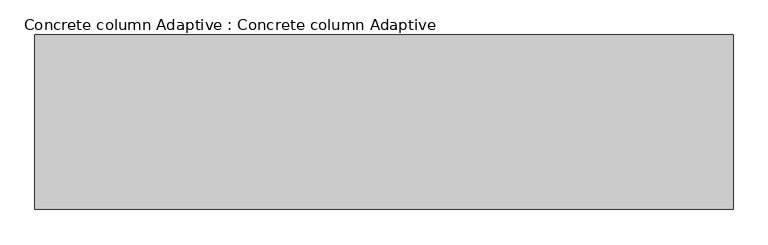
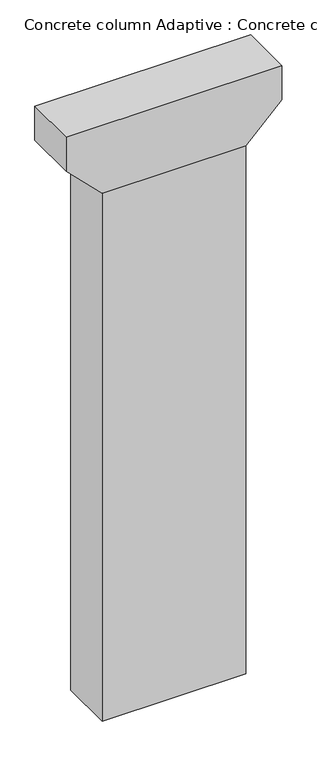
"""IFC4 building model written with IfcOpenShell, lengths in millimetres: proxy geometry, Concrete column Adaptive : Concrete column Adaptive."""

from ifc_helpers import new_model, si_unit, frame, origin, origin_with_axes, place, context, project, spatial, polyline, outline, extrude, source, transform, mapped, element, save


def concrete_column_adaptive_concrete_column_adaptive_b0f9f52a(model_context):
    return source(origin(), model_context, "Body", "SweptSolid", [
        extrude(outline(polyline([(35017.0, 6000.0), (35017.0, -6000.0), (33017.0, -6000.0), (31017.0, -4000.0), (31017.0, 4000.0), (33017.0, 6000.0), (35017.0, 6000.0)])), frame((0.0, -1500.0, 0.0), z_axis=(0.0, 1.0, 0.0), x_axis=(0.0, 0.0, 1.0)), (0.0, 0.0, 1.0), 3000.0),
        extrude(outline(polyline([(-4000.0, -1500.0), (-4000.0, 1500.0), (4000.0, 1500.0), (4000.0, -1500.0), (-4000.0, -1500.0)])), origin_with_axes(), (0.0, 0.0, 1.0), 31017.0),
    ])


if __name__ == "__main__":
    model = new_model("IFC4")
    model_context = context("Model", 3, world=origin())
    ifc_project = project(units=[si_unit("LENGTHUNIT", "METRE", prefix="MILLI")], contexts=[model_context])
    site = spatial("IfcSite", under=ifc_project)
    building = spatial("IfcBuilding", under=site)
    placement = place(None, origin())
    concrete_column_adaptive_concrete_column_adaptive_shape = concrete_column_adaptive_concrete_column_adaptive_b0f9f52a(model_context)
    element("IfcBuildingElementProxy", 1, Name="Concrete column Adaptive : Concrete column Adaptive", ObjectType="Concrete column Adaptive : Concrete column Adaptive", at=placement, inside=building, context=model_context, shape_type="MappedRepresentation", body=[
        mapped(concrete_column_adaptive_concrete_column_adaptive_shape, transform((0.0, 0.0, 0.0), x_axis=(1.0, 0.0, 0.0), y_axis=(0.0, 1.0, 0.0), z_axis=(0.0, 0.0, 1.0))),
    ])
    save(model, "model.ifc")

# Revit data of these elements
# Type "Concrete column Adaptive : Concrete column Adaptive"
#   Height [instance default] = 30000 mm
#   Default Elevation = 0
# Element 1 (IfcBuildingElementProxy, "Concrete column Adaptive : Concrete column Adaptive")
#   Height = 31017 mm
